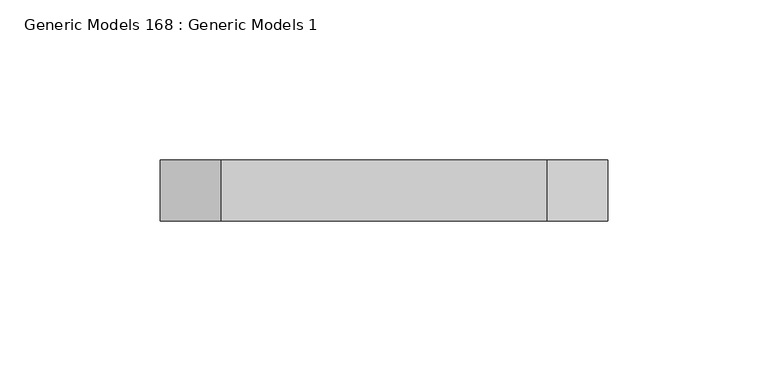
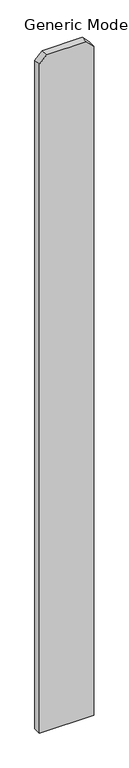
"""IFC4 building model written with IfcOpenShell, lengths in millimetres: proxy geometry, Generic Models 168 : Generic Models 1."""

import ifcopenshell
import ifcopenshell.guid

model = None  # the IFC model being written
_history = None  # IfcOwnerHistory: only IFC2X3 demands one
_inside = {}  # id of a spatial element -> (the spatial element, [elements in it])
_under = {}  # id of a project, library or spatial element -> (it, [spatial elements below it])
_declared = {}  # id of a project -> (the project, [libraries it declares])
_typed = {}  # id of a type object -> (the type object, [elements of that type])
_made_of = {}  # id of a material, layer set ... -> (it, [elements and type objects made of it])


def new_model(schema):
    """Start an empty IFC model of exactly this schema.

    Asked for "IFC4X3", IfcOpenShell would pick the latest addendum, in which some entities
    have other attributes; the version numbers below select the first issue.
    IFC2X3 requires an IfcOwnerHistory on every rooted entity: one is made here for all.
    """
    global model, _history
    if schema == "IFC4X3":
        model = ifcopenshell.file(schema_version=(4, 3, 0, 0))
    else:
        model = ifcopenshell.file(schema=schema)
    _inside.clear()
    _under.clear()
    _declared.clear()
    _typed.clear()
    _made_of.clear()
    _history = None
    if model.schema == "IFC2X3":
        org = make("IfcOrganization", Name="unknown")
        user = make(
            "IfcPersonAndOrganization",
            ThePerson=make("IfcPerson", FamilyName="unknown"),
            TheOrganization=org,
        )
        app = make(
            "IfcApplication",
            ApplicationDeveloper=org,
            Version="unknown",
            ApplicationFullName="unknown",
            ApplicationIdentifier="unknown",
        )
        _history = make(
            "IfcOwnerHistory",
            OwningUser=user,
            OwningApplication=app,
            ChangeAction="ADDED",
            CreationDate=0,
        )
    return model


def make(cls, **values):
    """One entity of the class cls with the attributes given. An attribute that is None is left unset."""
    return model.create_entity(
        cls, **{name: value for name, value in values.items() if value is not None}
    )


def rooted(cls, **values):
    """An entity with a GlobalId (a new one), such as an element, a storey or a relation."""
    return make(cls, GlobalId=ifcopenshell.guid.new(), OwnerHistory=_history, **values)


def si_unit(unit_type, name, prefix=None):
    """IfcSIUnit, for example si_unit("LENGTHUNIT", "METRE", prefix="MILLI")."""
    return make("IfcSIUnit", UnitType=unit_type, Prefix=prefix, Name=name)


def assignment(units):
    """IfcUnitAssignment: the units of a project."""
    return None if units is None else make("IfcUnitAssignment", Units=units)


def point(xyz):
    """IfcCartesianPoint."""
    return None if xyz is None else make("IfcCartesianPoint", Coordinates=xyz)


def direction(xyz):
    """IfcDirection."""
    return None if xyz is None else make("IfcDirection", DirectionRatios=xyz)


def frame(location, z_axis=None, x_axis=None):
    """IfcAxis2Placement3D, a coordinate frame: its origin and axes. An axis left out is left unset."""
    return make(
        "IfcAxis2Placement3D",
        Location=point(location),
        Axis=direction(z_axis),
        RefDirection=direction(x_axis),
    )


def origin():
    """The frame at (0, 0, 0) with its axes left unset."""
    return frame((0.0, 0.0, 0.0))


def place(relative_to, where):
    """IfcLocalPlacement: puts the frame where relative to a parent placement (None: the world)."""
    return make(
        "IfcLocalPlacement", PlacementRelTo=relative_to, RelativePlacement=where
    )


def context(
    kind, dimensions, precision=None, world=None, true_north=None, identifier=None
):
    """IfcGeometricRepresentationContext, for example the 3D "Model" context."""
    return make(
        "IfcGeometricRepresentationContext",
        ContextIdentifier=identifier,
        ContextType=kind,
        CoordinateSpaceDimension=dimensions,
        Precision=precision,
        WorldCoordinateSystem=world,
        TrueNorth=true_north,
    )


def project(units=None, contexts=None):
    """IfcProject with its units and contexts."""
    return rooted(
        "IfcProject",
        Name="project",
        RepresentationContexts=contexts,
        UnitsInContext=assignment(units),
    )


def spatial(cls, under=None, at=None, **own):
    """A site, building, storey or space (cls), placed at a placement, below another one or the project."""
    s = rooted(cls, ObjectPlacement=at, **own)
    if under is not None:
        _under.setdefault(under.id(), (under, []))[1].append(s)
    return s


def polyline(points):
    """IfcPolyline through the points."""
    return make("IfcPolyline", Points=[point(p) for p in points])


def outline(outer, holes=None, kind="AREA"):
    """IfcArbitraryClosedProfileDef: a profile drawn as a closed curve; with holes, ...WithVoids."""
    if holes is None:
        return make("IfcArbitraryClosedProfileDef", ProfileType=kind, OuterCurve=outer)
    return make(
        "IfcArbitraryProfileDefWithVoids",
        ProfileType=kind,
        OuterCurve=outer,
        InnerCurves=holes,
    )


def extrude(swept, where, along, depth):
    """IfcExtrudedAreaSolid: the profile swept, set in the frame where, extruded along a direction by depth."""
    return make(
        "IfcExtrudedAreaSolid",
        SweptArea=swept,
        Position=where,
        ExtrudedDirection=direction(along),
        Depth=depth,
    )


def shape(context_of_items, identifier, shape_type, items):
    """IfcShapeRepresentation: the items that make up one representation, for example the "Body"."""
    return make(
        "IfcShapeRepresentation",
        ContextOfItems=context_of_items,
        RepresentationIdentifier=identifier,
        RepresentationType=shape_type,
        Items=items,
    )


def source(mapping_origin, context_of_items, identifier, shape_type, items):
    """IfcRepresentationMap: a shape defined once, which mapped items show again and again."""
    return make(
        "IfcRepresentationMap",
        MappingOrigin=mapping_origin,
        MappedRepresentation=shape(context_of_items, identifier, shape_type, items),
    )


def transform(
    local_origin,
    x_axis=None,
    y_axis=None,
    z_axis=None,
    scale=None,
    scale2=None,
    scale3=None,
    uniform=True,
):
    """IfcCartesianTransformationOperator3D, or its non-uniform kind. x_axis, y_axis, z_axis: its Axis1, 2, 3."""
    if uniform:
        return make(
            "IfcCartesianTransformationOperator3D",
            Axis1=direction(x_axis),
            Axis2=direction(y_axis),
            LocalOrigin=point(local_origin),
            Scale=scale,
            Axis3=direction(z_axis),
        )
    return make(
        "IfcCartesianTransformationOperator3DnonUniform",
        Axis1=direction(x_axis),
        Axis2=direction(y_axis),
        LocalOrigin=point(local_origin),
        Scale=scale,
        Axis3=direction(z_axis),
        Scale2=scale2,
        Scale3=scale3,
    )


def mapped(mapping_source, mapping_target):
    """IfcMappedItem: shows the shape of a source again, moved by a transform."""
    return make(
        "IfcMappedItem", MappingSource=mapping_source, MappingTarget=mapping_target
    )


def made_of(thing, what):
    """Note that an element or type object is made of a material, layer set ...; save() writes the relation."""
    if what is not None:
        _made_of.setdefault(what.id(), (what, []))[1].append(thing)
    return thing


def element(
    cls,
    number,
    at=None,
    inside=None,
    cuts=None,
    type_object=None,
    material=None,
    context=None,
    identifier="Body",
    shape_type=None,
    held_by="IfcProductDefinitionShape",
    body=None,
    shapes=None,
    **own,
):
    """One element of the class cls, such as IfcWall. Its Tag is "e" and its number.

    at: its placement. inside: the storey or other place that contains it. cuts: it is an
    opening in that element (IfcRelVoidsElement). A single representation is given by context,
    identifier, shape_type and body (its items); several are given by shapes. held_by: the class
    of the entity that holds the representations. save() writes the other relations.
    """
    e = rooted(cls, Tag="e%d" % number, ObjectPlacement=at, **own)
    if body is not None:
        shapes = [shape(context, identifier, shape_type, body)]
    if shapes is not None:
        e.Representation = make(held_by, Representations=shapes)
    if inside is not None:
        _inside.setdefault(inside.id(), (inside, []))[1].append(e)
    if cuts is not None:
        rooted(
            "IfcRelVoidsElement", RelatingBuildingElement=cuts, RelatedOpeningElement=e
        )
    if type_object is not None:
        _typed.setdefault(type_object.id(), (type_object, []))[1].append(e)
    return made_of(e, material)


def aggregate(whole, parts):
    """IfcRelAggregates: a whole, such as a stair, and the parts it consists of."""
    return rooted("IfcRelAggregates", RelatingObject=whole, RelatedObjects=parts)


def save(model, path):
    """Write the relations noted so far, then the file.

    IfcRelAggregates (storeys below a building ...), IfcRelContainedInSpatialStructure (elements
    in a storey), IfcRelDefinesByType, IfcRelAssociatesMaterial and IfcRelDeclares: one each for
    every whole, place, type object, material and project.
    """
    for whole, parts in _under.values():
        aggregate(whole, parts)
    for where, things in _inside.values():
        rooted(
            "IfcRelContainedInSpatialStructure",
            RelatedElements=things,
            RelatingStructure=where,
        )
    for kind, things in _typed.values():
        rooted("IfcRelDefinesByType", RelatedObjects=things, RelatingType=kind)
    for what, things in _made_of.values():
        rooted("IfcRelAssociatesMaterial", RelatedObjects=things, RelatingMaterial=what)
    for by, libraries in _declared.values():
        rooted("IfcRelDeclares", RelatingContext=by, RelatedDefinitions=libraries)
    model.write(path)


def generic_models_168_generic_models_1_c133e3c9(model_context):
    return source(origin(), model_context, "Body", "SweptSolid", [
        extrude(outline(polyline([(76.2, 55599.0125), (1885.95, 55599.0125), (1905.0, 55579.9625), (1905.0, 55478.3625), (1885.95, 55459.3125), (76.2, 55459.3125), (76.2, 55599.0125)])), frame((0.0, 547.6875, 0.0), z_axis=(0.0, 1.0, 0.0), x_axis=(0.0, 0.0, 1.0)), (0.0, 0.0, 1.0), 19.05),
    ])


if __name__ == "__main__":
    model = new_model("IFC4")
    model_context = context("Model", 3, world=origin())
    ifc_project = project(units=[si_unit("LENGTHUNIT", "METRE", prefix="MILLI")], contexts=[model_context])
    site = spatial("IfcSite", under=ifc_project)
    building = spatial("IfcBuilding", under=site)
    placement = place(None, origin())
    generic_models_168_generic_models_1_shape = generic_models_168_generic_models_1_c133e3c9(model_context)
    element("IfcBuildingElementProxy", 1, Name="Generic Models 168 : Generic Models 1", ObjectType="Generic Models 168 : Generic Models 1", at=placement, inside=building, context=model_context, shape_type="MappedRepresentation", body=[
        mapped(generic_models_168_generic_models_1_shape, transform((0.0, 0.0, 0.0), x_axis=(1.0, 0.0, 0.0), y_axis=(0.0, 1.0, 0.0), z_axis=(0.0, 0.0, 1.0))),
    ])
    save(model, "model.ifc")

# Revit data of these elements
# Element 1 (IfcBuildingElementProxy, "Generic Models 168 : Generic Models 1")
#   Materials on its faces: "VERTICAL 1X6 CEDAR PLANKS W/ CLEAR WOOD SEALER"
# Materials
#   "VERTICAL 1X6 CEDAR PLANKS W/ CLEAR WOOD SEALER": class "Wood", colour RGB 234 198 147, transparency 0, Description = "Pinus Echinata", Cost = 0
